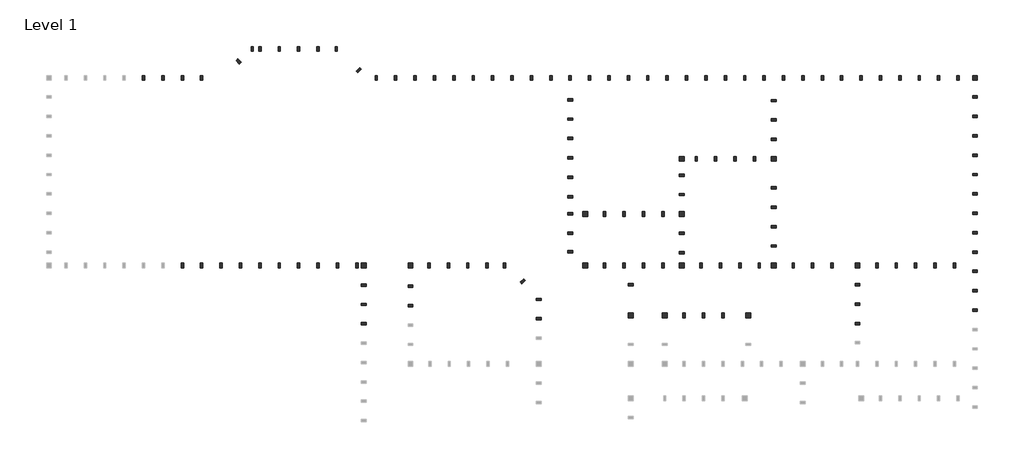
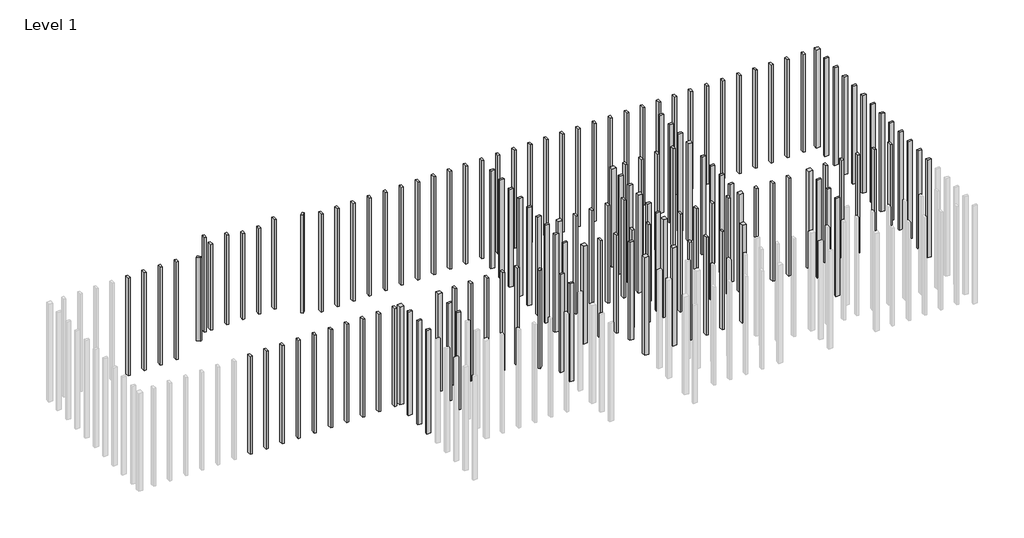
# One storey, part 2 of 2: 143 columns.
"""IFC4 building model written with IfcOpenShell, lengths in millimetres."""

import ifcopenshell
import ifcopenshell.guid

model = None  # the IFC model being written
_history = None  # IfcOwnerHistory: only IFC2X3 demands one
_inside = {}  # id of a spatial element -> (the spatial element, [elements in it])
_under = {}  # id of a project, library or spatial element -> (it, [spatial elements below it])
_declared = {}  # id of a project -> (the project, [libraries it declares])
_typed = {}  # id of a type object -> (the type object, [elements of that type])
_made_of = {}  # id of a material, layer set ... -> (it, [elements and type objects made of it])


def new_model(schema):
    """Start an empty IFC model of exactly this schema.

    Asked for "IFC4X3", IfcOpenShell would pick the latest addendum, in which some entities
    have other attributes; the version numbers below select the first issue.
    IFC2X3 requires an IfcOwnerHistory on every rooted entity: one is made here for all.
    """
    global model, _history
    if schema == "IFC4X3":
        model = ifcopenshell.file(schema_version=(4, 3, 0, 0))
    else:
        model = ifcopenshell.file(schema=schema)
    _inside.clear()
    _under.clear()
    _declared.clear()
    _typed.clear()
    _made_of.clear()
    _history = None
    if model.schema == "IFC2X3":
        org = make("IfcOrganization", Name="unknown")
        user = make(
            "IfcPersonAndOrganization",
            ThePerson=make("IfcPerson", FamilyName="unknown"),
            TheOrganization=org,
        )
        app = make(
            "IfcApplication",
            ApplicationDeveloper=org,
            Version="unknown",
            ApplicationFullName="unknown",
            ApplicationIdentifier="unknown",
        )
        _history = make(
            "IfcOwnerHistory",
            OwningUser=user,
            OwningApplication=app,
            ChangeAction="ADDED",
            CreationDate=0,
        )
    return model


def make(cls, **values):
    """One entity of the class cls with the attributes given. An attribute that is None is left unset."""
    return model.create_entity(
        cls, **{name: value for name, value in values.items() if value is not None}
    )


def rooted(cls, **values):
    """An entity with a GlobalId (a new one), such as an element, a storey or a relation."""
    return make(cls, GlobalId=ifcopenshell.guid.new(), OwnerHistory=_history, **values)


def si_unit(unit_type, name, prefix=None):
    """IfcSIUnit, for example si_unit("LENGTHUNIT", "METRE", prefix="MILLI")."""
    return make("IfcSIUnit", UnitType=unit_type, Prefix=prefix, Name=name)


def assignment(units):
    """IfcUnitAssignment: the units of a project."""
    return None if units is None else make("IfcUnitAssignment", Units=units)


def point(xyz):
    """IfcCartesianPoint."""
    return None if xyz is None else make("IfcCartesianPoint", Coordinates=xyz)


def direction(xyz):
    """IfcDirection."""
    return None if xyz is None else make("IfcDirection", DirectionRatios=xyz)


def frame(location, z_axis=None, x_axis=None):
    """IfcAxis2Placement3D, a coordinate frame: its origin and axes. An axis left out is left unset."""
    return make(
        "IfcAxis2Placement3D",
        Location=point(location),
        Axis=direction(z_axis),
        RefDirection=direction(x_axis),
    )


def origin():
    """The frame at (0, 0, 0) with its axes left unset."""
    return frame((0.0, 0.0, 0.0))


def origin_with_axes():
    """The frame at (0, 0, 0) with the z axis (0, 0, 1) and the x axis (1, 0, 0) written out."""
    return frame((0.0, 0.0, 0.0), z_axis=(0.0, 0.0, 1.0), x_axis=(1.0, 0.0, 0.0))


def place(relative_to, where):
    """IfcLocalPlacement: puts the frame where relative to a parent placement (None: the world)."""
    return make(
        "IfcLocalPlacement", PlacementRelTo=relative_to, RelativePlacement=where
    )


def context(
    kind, dimensions, precision=None, world=None, true_north=None, identifier=None
):
    """IfcGeometricRepresentationContext, for example the 3D "Model" context."""
    return make(
        "IfcGeometricRepresentationContext",
        ContextIdentifier=identifier,
        ContextType=kind,
        CoordinateSpaceDimension=dimensions,
        Precision=precision,
        WorldCoordinateSystem=world,
        TrueNorth=true_north,
    )


def project(units=None, contexts=None):
    """IfcProject with its units and contexts."""
    return rooted(
        "IfcProject",
        Name="project",
        RepresentationContexts=contexts,
        UnitsInContext=assignment(units),
    )


def spatial(cls, under=None, at=None, **own):
    """A site, building, storey or space (cls), placed at a placement, below another one or the project."""
    s = rooted(cls, ObjectPlacement=at, **own)
    if under is not None:
        _under.setdefault(under.id(), (under, []))[1].append(s)
    return s


def polyline(points):
    """IfcPolyline through the points."""
    return make("IfcPolyline", Points=[point(p) for p in points])


def outline(outer, holes=None, kind="AREA"):
    """IfcArbitraryClosedProfileDef: a profile drawn as a closed curve; with holes, ...WithVoids."""
    if holes is None:
        return make("IfcArbitraryClosedProfileDef", ProfileType=kind, OuterCurve=outer)
    return make(
        "IfcArbitraryProfileDefWithVoids",
        ProfileType=kind,
        OuterCurve=outer,
        InnerCurves=holes,
    )


def extrude(swept, where, along, depth):
    """IfcExtrudedAreaSolid: the profile swept, set in the frame where, extruded along a direction by depth."""
    return make(
        "IfcExtrudedAreaSolid",
        SweptArea=swept,
        Position=where,
        ExtrudedDirection=direction(along),
        Depth=depth,
    )


def shape(context_of_items, identifier, shape_type, items):
    """IfcShapeRepresentation: the items that make up one representation, for example the "Body"."""
    return make(
        "IfcShapeRepresentation",
        ContextOfItems=context_of_items,
        RepresentationIdentifier=identifier,
        RepresentationType=shape_type,
        Items=items,
    )


def source(mapping_origin, context_of_items, identifier, shape_type, items):
    """IfcRepresentationMap: a shape defined once, which mapped items show again and again."""
    return make(
        "IfcRepresentationMap",
        MappingOrigin=mapping_origin,
        MappedRepresentation=shape(context_of_items, identifier, shape_type, items),
    )


def transform(
    local_origin,
    x_axis=None,
    y_axis=None,
    z_axis=None,
    scale=None,
    scale2=None,
    scale3=None,
    uniform=True,
):
    """IfcCartesianTransformationOperator3D, or its non-uniform kind. x_axis, y_axis, z_axis: its Axis1, 2, 3."""
    if uniform:
        return make(
            "IfcCartesianTransformationOperator3D",
            Axis1=direction(x_axis),
            Axis2=direction(y_axis),
            LocalOrigin=point(local_origin),
            Scale=scale,
            Axis3=direction(z_axis),
        )
    return make(
        "IfcCartesianTransformationOperator3DnonUniform",
        Axis1=direction(x_axis),
        Axis2=direction(y_axis),
        LocalOrigin=point(local_origin),
        Scale=scale,
        Axis3=direction(z_axis),
        Scale2=scale2,
        Scale3=scale3,
    )


def mapped(mapping_source, mapping_target):
    """IfcMappedItem: shows the shape of a source again, moved by a transform."""
    return make(
        "IfcMappedItem", MappingSource=mapping_source, MappingTarget=mapping_target
    )


def made_of(thing, what):
    """Note that an element or type object is made of a material, layer set ...; save() writes the relation."""
    if what is not None:
        _made_of.setdefault(what.id(), (what, []))[1].append(thing)
    return thing


def element(
    cls,
    number,
    at=None,
    inside=None,
    cuts=None,
    type_object=None,
    material=None,
    context=None,
    identifier="Body",
    shape_type=None,
    held_by="IfcProductDefinitionShape",
    body=None,
    shapes=None,
    **own,
):
    """One element of the class cls, such as IfcWall. Its Tag is "e" and its number.

    at: its placement. inside: the storey or other place that contains it. cuts: it is an
    opening in that element (IfcRelVoidsElement). A single representation is given by context,
    identifier, shape_type and body (its items); several are given by shapes. held_by: the class
    of the entity that holds the representations. save() writes the other relations.
    """
    e = rooted(cls, Tag="e%d" % number, ObjectPlacement=at, **own)
    if body is not None:
        shapes = [shape(context, identifier, shape_type, body)]
    if shapes is not None:
        e.Representation = make(held_by, Representations=shapes)
    if inside is not None:
        _inside.setdefault(inside.id(), (inside, []))[1].append(e)
    if cuts is not None:
        rooted(
            "IfcRelVoidsElement", RelatingBuildingElement=cuts, RelatedOpeningElement=e
        )
    if type_object is not None:
        _typed.setdefault(type_object.id(), (type_object, []))[1].append(e)
    return made_of(e, material)


def aggregate(whole, parts):
    """IfcRelAggregates: a whole, such as a stair, and the parts it consists of."""
    return rooted("IfcRelAggregates", RelatingObject=whole, RelatedObjects=parts)


def save(model, path):
    """Write the relations noted so far, then the file.

    IfcRelAggregates (storeys below a building ...), IfcRelContainedInSpatialStructure (elements
    in a storey), IfcRelDefinesByType, IfcRelAssociatesMaterial and IfcRelDeclares: one each for
    every whole, place, type object, material and project.
    """
    for whole, parts in _under.values():
        aggregate(whole, parts)
    for where, things in _inside.values():
        rooted(
            "IfcRelContainedInSpatialStructure",
            RelatedElements=things,
            RelatingStructure=where,
        )
    for kind, things in _typed.values():
        rooted("IfcRelDefinesByType", RelatedObjects=things, RelatingType=kind)
    for what, things in _made_of.values():
        rooted("IfcRelAssociatesMaterial", RelatedObjects=things, RelatingMaterial=what)
    for by, libraries in _declared.values():
        rooted("IfcRelDeclares", RelatingContext=by, RelatedDefinitions=libraries)
    model.write(path)


def timber_column_65e54e3c(model_context):
    return source(origin(), model_context, "Body", "SweptSolid", [
        extrude(outline(polyline([(25.4, 50.8), (25.4, -50.8), (-25.4, -50.8), (-25.4, 50.8), (25.4, 50.8)])), frame((0.0, 0.0, 50.8), z_axis=(0.0, 0.0, 1.0), x_axis=(1.0, 0.0, 0.0)), (0.0, 0.0, 1.0), 2616.2),
    ])


def timber_column_b7e6a7b9(model_context):
    return source(origin(), model_context, "Body", "SweptSolid", [
        extrude(outline(polyline([(50.8, 50.8), (50.8, -50.8), (-50.8, -50.8), (-50.8, 50.8), (50.8, 50.8)])), frame((0.0, 0.0, 50.8), z_axis=(0.0, 0.0, 1.0), x_axis=(1.0, 0.0, 0.0)), (0.0, 0.0, 1.0), 2616.2),
    ])


def timber_column_c014de30(model_context):
    return source(origin(), model_context, "Body", "SweptSolid", [
        extrude(outline(polyline([(25.4, -50.8), (-25.4, -50.8), (-25.4, 50.8), (25.4, 50.8), (25.4, -50.8)])), frame((0.0, 0.0, 50.8), z_axis=(0.0, 0.0, 1.0), x_axis=(1.0, 0.0, 0.0)), (0.0, 0.0, 1.0), 2616.2),
    ])


def timber_column_7e99ce9a(model_context):
    return source(origin(), model_context, "Body", "SweptSolid", [
        extrude(outline(polyline([(25.4, 50.8), (25.4, -50.8), (-25.4, -50.8), (-25.4, 50.8), (25.4, 50.8)])), origin_with_axes(), (0.0, 0.0, 1.0), 2768.6),
    ])


def timber_column_b6a9144e(model_context):
    return source(origin(), model_context, "Body", "SweptSolid", [
        extrude(outline(polyline([(25.4, 50.8), (25.4, -50.8), (-25.4, -50.8), (-25.4, 50.8), (25.4, 50.8)])), frame((0.0, 0.0, 50.8), z_axis=(0.0, 0.0, 1.0), x_axis=(1.0, 0.0, 0.0)), (0.0, 0.0, 1.0), 2290.1727203),
    ])


model = new_model("IFC4")

# Units and contexts
model_context = context("Model", 3, world=origin())
ifc_project = project(units=[si_unit("LENGTHUNIT", "METRE", prefix="MILLI")], contexts=[model_context])

# Site, building, storey
site = spatial("IfcSite", under=ifc_project)
building = spatial("IfcBuilding", under=site)
storey = spatial("IfcBuildingStorey", under=building, Name="Level 1", Elevation=0.0)

# Columns
placement = place(None, origin())
element("IfcColumn", 1, ObjectType="Timber-Column", at=placement, inside=storey, context=model_context, shape_type="SweptSolid", body=[
    extrude(outline(polyline([(-13305.414829, 5817.3284114), (-13305.414829, 5715.7284114), (-13356.214829, 5715.7284114), (-13356.214829, 5817.3284114), (-13305.414829, 5817.3284114)])), frame((0.0, 0.0, 50.8), z_axis=(0.0, 0.0, 1.0), x_axis=(1.0, 0.0, 0.0)), (0.0, 0.0, 1.0), 2290.1727203),
])
element("IfcColumn", 2, ObjectType="Timber-Column", at=placement, inside=storey, context=model_context, shape_type="SweptSolid", body=[
    extrude(outline(polyline([(-12899.014829, 5817.3284114), (-12899.014829, 5715.7284114), (-12949.814829, 5715.7284114), (-12949.814829, 5817.3284114), (-12899.014829, 5817.3284114)])), frame((0.0, 0.0, 50.8), z_axis=(0.0, 0.0, 1.0), x_axis=(1.0, 0.0, 0.0)), (0.0, 0.0, 1.0), 2391.7727203),
])
element("IfcColumn", 3, ObjectType="Timber-Column", at=placement, inside=storey, context=model_context, shape_type="SweptSolid", body=[
    extrude(outline(polyline([(-13793.9590772, 5557.3841632), (-13722.1170283, 5485.5421142), (-13758.0380528, 5449.6210897), (-13829.8801017, 5521.4631387), (-13793.9590772, 5557.3841632)])), frame((0.0, 0.0, 50.8), z_axis=(0.0, 0.0, 1.0), x_axis=(1.0, 0.0, 0.0)), (0.0, 0.0, 1.0), 2235.2),
])
element("IfcColumn", 4, ObjectType="Timber-Column", at=placement, inside=storey, context=model_context, shape_type="SweptSolid", body=[
    extrude(outline(polyline([(-13464.8030362, 5817.3284114), (-13464.8030362, 5715.7284114), (-13515.6030362, 5715.7284114), (-13515.6030362, 5817.3284114), (-13464.8030362, 5817.3284114)])), frame((0.0, 0.0, 50.8), z_axis=(0.0, 0.0, 1.0), x_axis=(1.0, 0.0, 0.0)), (0.0, 0.0, 1.0), 2528.0077467),
])
element("IfcColumn", 5, ObjectType="Timber-Column", at=placement, inside=storey, context=model_context, shape_type="SweptSolid", body=[
    extrude(outline(polyline([(-11705.214829, 5817.3284114), (-11705.214829, 5715.7284114), (-11756.014829, 5715.7284114), (-11756.014829, 5817.3284114), (-11705.214829, 5817.3284114)])), frame((0.0, 0.0, 50.8), z_axis=(0.0, 0.0, 1.0), x_axis=(1.0, 0.0, 0.0)), (0.0, 0.0, 1.0), 2391.7727203),
])
timber_column_shape = timber_column_65e54e3c(model_context)
element("IfcColumn", 6, ObjectType="Timber-Column", at=placement, inside=storey, context=model_context, shape_type="MappedRepresentation", body=[
    mapped(timber_column_shape, transform((-15769.214829, 5156.9284114, 0.0), x_axis=(1.0, 0.0, 0.0), y_axis=(0.0, 1.0, 0.0), z_axis=(0.0, 0.0, 1.0))),
])
element("IfcColumn", 7, ObjectType="Timber-Column", at=placement, inside=storey, context=model_context, shape_type="MappedRepresentation", body=[
    mapped(timber_column_shape, transform((-15362.814829, 5156.9284114, 0.0), x_axis=(1.0, 0.0, 0.0), y_axis=(0.0, 1.0, 0.0), z_axis=(0.0, 0.0, 1.0))),
])
element("IfcColumn", 8, ObjectType="Timber-Column", at=placement, inside=storey, context=model_context, shape_type="MappedRepresentation", body=[
    mapped(timber_column_shape, transform((-14956.414829, 5156.9284114, 0.0), x_axis=(1.0, 0.0, 0.0), y_axis=(0.0, 1.0, 0.0), z_axis=(0.0, 0.0, 1.0))),
])
element("IfcColumn", 9, ObjectType="Timber-Column", at=placement, inside=storey, context=model_context, shape_type="MappedRepresentation", body=[
    mapped(timber_column_shape, transform((-14550.014829, 5156.9284114, 0.0), x_axis=(1.0, 0.0, 0.0), y_axis=(0.0, 1.0, 0.0), z_axis=(0.0, 0.0, 1.0))),
])
element("IfcColumn", 10, ObjectType="Timber-Column", at=placement, inside=storey, context=model_context, shape_type="MappedRepresentation", body=[
    mapped(timber_column_shape, transform((-10892.414829, 5156.9284114, 0.0), x_axis=(1.0, 0.0, 0.0), y_axis=(0.0, 1.0, 0.0), z_axis=(0.0, 0.0, 1.0))),
])
element("IfcColumn", 11, ObjectType="Timber-Column", at=placement, inside=storey, context=model_context, shape_type="MappedRepresentation", body=[
    mapped(timber_column_shape, transform((-10486.014829, 5156.9284114, 0.0), x_axis=(1.0, 0.0, 0.0), y_axis=(0.0, 1.0, 0.0), z_axis=(0.0, 0.0, 1.0))),
])
element("IfcColumn", 12, ObjectType="Timber-Column", at=placement, inside=storey, context=model_context, shape_type="MappedRepresentation", body=[
    mapped(timber_column_shape, transform((-10079.614829, 5156.9284114, 0.0), x_axis=(1.0, 0.0, 0.0), y_axis=(0.0, 1.0, 0.0), z_axis=(0.0, 0.0, 1.0))),
])
element("IfcColumn", 13, ObjectType="Timber-Column", at=placement, inside=storey, context=model_context, shape_type="MappedRepresentation", body=[
    mapped(timber_column_shape, transform((-9673.214829, 5156.9284114, 0.0), x_axis=(1.0, 0.0, 0.0), y_axis=(0.0, 1.0, 0.0), z_axis=(0.0, 0.0, 1.0))),
])
element("IfcColumn", 14, ObjectType="Timber-Column", at=placement, inside=storey, context=model_context, shape_type="MappedRepresentation", body=[
    mapped(timber_column_shape, transform((-9266.814829, 5156.9284114, 0.0), x_axis=(1.0, 0.0, 0.0), y_axis=(0.0, 1.0, 0.0), z_axis=(0.0, 0.0, 1.0))),
])
element("IfcColumn", 15, ObjectType="Timber-Column", at=placement, inside=storey, context=model_context, shape_type="MappedRepresentation", body=[
    mapped(timber_column_shape, transform((-8860.414829, 5156.9284114, 0.0), x_axis=(1.0, 0.0, 0.0), y_axis=(0.0, 1.0, 0.0), z_axis=(0.0, 0.0, 1.0))),
])
element("IfcColumn", 16, ObjectType="Timber-Column", at=placement, inside=storey, context=model_context, shape_type="MappedRepresentation", body=[
    mapped(timber_column_shape, transform((-8454.014829, 5156.9284114, 0.0), x_axis=(1.0, 0.0, 0.0), y_axis=(0.0, 1.0, 0.0), z_axis=(0.0, 0.0, 1.0))),
])
element("IfcColumn", 17, ObjectType="Timber-Column", at=placement, inside=storey, context=model_context, shape_type="MappedRepresentation", body=[
    mapped(timber_column_shape, transform((-8047.614829, 5156.9284114, 0.0), x_axis=(1.0, 0.0, 0.0), y_axis=(0.0, 1.0, 0.0), z_axis=(0.0, 0.0, 1.0))),
])
element("IfcColumn", 18, ObjectType="Timber-Column", at=placement, inside=storey, context=model_context, shape_type="MappedRepresentation", body=[
    mapped(timber_column_shape, transform((-7641.214829, 5156.9284114, 0.0), x_axis=(1.0, 0.0, 0.0), y_axis=(0.0, 1.0, 0.0), z_axis=(0.0, 0.0, 1.0))),
])
element("IfcColumn", 19, ObjectType="Timber-Column", at=placement, inside=storey, context=model_context, shape_type="MappedRepresentation", body=[
    mapped(timber_column_shape, transform((-7234.814829, 5156.9284114, 0.0), x_axis=(1.0, 0.0, 0.0), y_axis=(0.0, 1.0, 0.0), z_axis=(0.0, 0.0, 1.0))),
])
element("IfcColumn", 20, ObjectType="Timber-Column", at=placement, inside=storey, context=model_context, shape_type="MappedRepresentation", body=[
    mapped(timber_column_shape, transform((-6828.414829, 5156.9284114, 0.0), x_axis=(1.0, 0.0, 0.0), y_axis=(0.0, 1.0, 0.0), z_axis=(0.0, 0.0, 1.0))),
])
element("IfcColumn", 21, ObjectType="Timber-Column", at=placement, inside=storey, context=model_context, shape_type="MappedRepresentation", body=[
    mapped(timber_column_shape, transform((-6422.014829, 5156.9284114, 0.0), x_axis=(1.0, 0.0, 0.0), y_axis=(0.0, 1.0, 0.0), z_axis=(0.0, 0.0, 1.0))),
])
element("IfcColumn", 22, ObjectType="Timber-Column", at=placement, inside=storey, context=model_context, shape_type="MappedRepresentation", body=[
    mapped(timber_column_shape, transform((-6015.614829, 5156.9284114, 0.0), x_axis=(1.0, 0.0, 0.0), y_axis=(0.0, 1.0, 0.0), z_axis=(0.0, 0.0, 1.0))),
])
element("IfcColumn", 23, ObjectType="Timber-Column", at=placement, inside=storey, context=model_context, shape_type="MappedRepresentation", body=[
    mapped(timber_column_shape, transform((-5609.214829, 5156.9284114, 0.0), x_axis=(1.0, 0.0, 0.0), y_axis=(0.0, 1.0, 0.0), z_axis=(0.0, 0.0, 1.0))),
])
element("IfcColumn", 24, ObjectType="Timber-Column", at=placement, inside=storey, context=model_context, shape_type="MappedRepresentation", body=[
    mapped(timber_column_shape, transform((-5202.814829, 5156.9284114, 0.0), x_axis=(1.0, 0.0, 0.0), y_axis=(0.0, 1.0, 0.0), z_axis=(0.0, 0.0, 1.0))),
])
element("IfcColumn", 25, ObjectType="Timber-Column", at=placement, inside=storey, context=model_context, shape_type="MappedRepresentation", body=[
    mapped(timber_column_shape, transform((-4796.414829, 5156.9284114, 0.0), x_axis=(1.0, 0.0, 0.0), y_axis=(0.0, 1.0, 0.0), z_axis=(0.0, 0.0, 1.0))),
])
element("IfcColumn", 26, ObjectType="Timber-Column", at=placement, inside=storey, context=model_context, shape_type="MappedRepresentation", body=[
    mapped(timber_column_shape, transform((-4390.014829, 5156.9284114, 0.0), x_axis=(1.0, 0.0, 0.0), y_axis=(0.0, 1.0, 0.0), z_axis=(0.0, 0.0, 1.0))),
])
element("IfcColumn", 27, ObjectType="Timber-Column", at=placement, inside=storey, context=model_context, shape_type="MappedRepresentation", body=[
    mapped(timber_column_shape, transform((-3983.614829, 5156.9284114, 0.0), x_axis=(1.0, 0.0, 0.0), y_axis=(0.0, 1.0, 0.0), z_axis=(0.0, 0.0, 1.0))),
])
element("IfcColumn", 28, ObjectType="Timber-Column", at=placement, inside=storey, context=model_context, shape_type="MappedRepresentation", body=[
    mapped(timber_column_shape, transform((-3577.214829, 5156.9284114, 0.0), x_axis=(1.0, 0.0, 0.0), y_axis=(0.0, 1.0, 0.0), z_axis=(0.0, 0.0, 1.0))),
])
element("IfcColumn", 29, ObjectType="Timber-Column", at=placement, inside=storey, context=model_context, shape_type="MappedRepresentation", body=[
    mapped(timber_column_shape, transform((-3170.814829, 5156.9284114, 0.0), x_axis=(1.0, 0.0, 0.0), y_axis=(0.0, 1.0, 0.0), z_axis=(0.0, 0.0, 1.0))),
])
element("IfcColumn", 30, ObjectType="Timber-Column", at=placement, inside=storey, context=model_context, shape_type="MappedRepresentation", body=[
    mapped(timber_column_shape, transform((-2764.414829, 5156.9284114, 0.0), x_axis=(1.0, 0.0, 0.0), y_axis=(0.0, 1.0, 0.0), z_axis=(0.0, 0.0, 1.0))),
])
element("IfcColumn", 31, ObjectType="Timber-Column", at=placement, inside=storey, context=model_context, shape_type="MappedRepresentation", body=[
    mapped(timber_column_shape, transform((-2358.014829, 5156.9284114, 0.0), x_axis=(1.0, 0.0, 0.0), y_axis=(0.0, 1.0, 0.0), z_axis=(0.0, 0.0, 1.0))),
])
element("IfcColumn", 32, ObjectType="Timber-Column", at=placement, inside=storey, context=model_context, shape_type="MappedRepresentation", body=[
    mapped(timber_column_shape, transform((-1951.614829, 5156.9284114, 0.0), x_axis=(1.0, 0.0, 0.0), y_axis=(0.0, 1.0, 0.0), z_axis=(0.0, 0.0, 1.0))),
])
element("IfcColumn", 33, ObjectType="Timber-Column", at=placement, inside=storey, context=model_context, shape_type="MappedRepresentation", body=[
    mapped(timber_column_shape, transform((-1545.214829, 5156.9284114, 0.0), x_axis=(1.0, 0.0, 0.0), y_axis=(0.0, 1.0, 0.0), z_axis=(0.0, 0.0, 1.0))),
])
element("IfcColumn", 34, ObjectType="Timber-Column", at=placement, inside=storey, context=model_context, shape_type="MappedRepresentation", body=[
    mapped(timber_column_shape, transform((-1138.814829, 5156.9284114, 0.0), x_axis=(1.0, 0.0, 0.0), y_axis=(0.0, 1.0, 0.0), z_axis=(0.0, 0.0, 1.0))),
])
element("IfcColumn", 35, ObjectType="Timber-Column", at=placement, inside=storey, context=model_context, shape_type="MappedRepresentation", body=[
    mapped(timber_column_shape, transform((-732.414829, 5156.9284114, 0.0), x_axis=(1.0, 0.0, 0.0), y_axis=(0.0, 1.0, 0.0), z_axis=(0.0, 0.0, 1.0))),
])
element("IfcColumn", 36, ObjectType="Timber-Column", at=placement, inside=storey, context=model_context, shape_type="MappedRepresentation", body=[
    mapped(timber_column_shape, transform((-326.014829, 5156.9284114, 0.0), x_axis=(1.0, 0.0, 0.0), y_axis=(0.0, 1.0, 0.0), z_axis=(0.0, 0.0, 1.0))),
])
element("IfcColumn", 37, ObjectType="Timber-Column", at=placement, inside=storey, context=model_context, shape_type="MappedRepresentation", body=[
    mapped(timber_column_shape, transform((80.385171, 5156.9284114, 0.0), x_axis=(1.0, 0.0, 0.0), y_axis=(0.0, 1.0, 0.0), z_axis=(0.0, 0.0, 1.0))),
])
element("IfcColumn", 38, ObjectType="Timber-Column", at=placement, inside=storey, context=model_context, shape_type="MappedRepresentation", body=[
    mapped(timber_column_shape, transform((486.785171, 5156.9284114, 0.0), x_axis=(1.0, 0.0, 0.0), y_axis=(0.0, 1.0, 0.0), z_axis=(0.0, 0.0, 1.0))),
])
element("IfcColumn", 39, ObjectType="Timber-Column", at=placement, inside=storey, context=model_context, shape_type="MappedRepresentation", body=[
    mapped(timber_column_shape, transform((893.185171, 5156.9284114, 0.0), x_axis=(1.0, 0.0, 0.0), y_axis=(0.0, 1.0, 0.0), z_axis=(0.0, 0.0, 1.0))),
])
element("IfcColumn", 40, ObjectType="Timber-Column", at=placement, inside=storey, context=model_context, shape_type="MappedRepresentation", body=[
    mapped(timber_column_shape, transform((1299.585171, 5156.9284114, 0.0), x_axis=(1.0, 0.0, 0.0), y_axis=(0.0, 1.0, 0.0), z_axis=(0.0, 0.0, 1.0))),
])
element("IfcColumn", 41, ObjectType="Timber-Column", at=placement, inside=storey, context=model_context, shape_type="MappedRepresentation", body=[
    mapped(timber_column_shape, transform((-11298.814829, 1226.2784114, 0.0), x_axis=(1.0, 0.0, 0.0), y_axis=(0.0, 1.0, 0.0), z_axis=(0.0, 0.0, 1.0))),
])
element("IfcColumn", 42, ObjectType="Timber-Column", at=placement, inside=storey, context=model_context, shape_type="MappedRepresentation", body=[
    mapped(timber_column_shape, transform((-11705.214829, 1226.2784114, 0.0), x_axis=(1.0, 0.0, 0.0), y_axis=(0.0, 1.0, 0.0), z_axis=(0.0, 0.0, 1.0))),
])
element("IfcColumn", 43, ObjectType="Timber-Column", at=placement, inside=storey, context=model_context, shape_type="MappedRepresentation", body=[
    mapped(timber_column_shape, transform((-12111.614829, 1226.2784114, 0.0), x_axis=(1.0, 0.0, 0.0), y_axis=(0.0, 1.0, 0.0), z_axis=(0.0, 0.0, 1.0))),
])
element("IfcColumn", 44, ObjectType="Timber-Column", at=placement, inside=storey, context=model_context, shape_type="MappedRepresentation", body=[
    mapped(timber_column_shape, transform((-12518.014829, 1226.2784114, 0.0), x_axis=(1.0, 0.0, 0.0), y_axis=(0.0, 1.0, 0.0), z_axis=(0.0, 0.0, 1.0))),
])
element("IfcColumn", 45, ObjectType="Timber-Column", at=placement, inside=storey, context=model_context, shape_type="MappedRepresentation", body=[
    mapped(timber_column_shape, transform((-12924.414829, 1226.2784114, 0.0), x_axis=(1.0, 0.0, 0.0), y_axis=(0.0, 1.0, 0.0), z_axis=(0.0, 0.0, 1.0))),
])
element("IfcColumn", 46, ObjectType="Timber-Column", at=placement, inside=storey, context=model_context, shape_type="MappedRepresentation", body=[
    mapped(timber_column_shape, transform((-13330.814829, 1226.2784114, 0.0), x_axis=(1.0, 0.0, 0.0), y_axis=(0.0, 1.0, 0.0), z_axis=(0.0, 0.0, 1.0))),
])
element("IfcColumn", 47, ObjectType="Timber-Column", at=placement, inside=storey, context=model_context, shape_type="MappedRepresentation", body=[
    mapped(timber_column_shape, transform((-13737.214829, 1226.2784114, 0.0), x_axis=(1.0, 0.0, 0.0), y_axis=(0.0, 1.0, 0.0), z_axis=(0.0, 0.0, 1.0))),
])
element("IfcColumn", 48, ObjectType="Timber-Column", at=placement, inside=storey, context=model_context, shape_type="MappedRepresentation", body=[
    mapped(timber_column_shape, transform((-14143.614829, 1226.2784114, 0.0), x_axis=(1.0, 0.0, 0.0), y_axis=(0.0, 1.0, 0.0), z_axis=(0.0, 0.0, 1.0))),
])
element("IfcColumn", 49, ObjectType="Timber-Column", at=placement, inside=storey, context=model_context, shape_type="MappedRepresentation", body=[
    mapped(timber_column_shape, transform((-14550.014829, 1226.2784114, 0.0), x_axis=(1.0, 0.0, 0.0), y_axis=(0.0, 1.0, 0.0), z_axis=(0.0, 0.0, 1.0))),
])
element("IfcColumn", 50, ObjectType="Timber-Column", at=placement, inside=storey, context=model_context, shape_type="MappedRepresentation", body=[
    mapped(timber_column_shape, transform((-14956.414829, 1226.2784114, 0.0), x_axis=(1.0, 0.0, 0.0), y_axis=(0.0, 1.0, 0.0), z_axis=(0.0, 0.0, 1.0))),
])
element("IfcColumn", 51, ObjectType="Timber-Column", at=placement, inside=storey, context=model_context, shape_type="MappedRepresentation", body=[
    mapped(timber_column_shape, transform((-11259.6474151, 5320.9609974, 0.0), x_axis=(0.7071067811865546, -0.7071067811865406, 0.0), y_axis=(0.7071067811865406, 0.7071067811865546, 0.0), z_axis=(0.0, 0.0, 1.0))),
])
element("IfcColumn", 52, ObjectType="Timber-Column", at=placement, inside=storey, context=model_context, shape_type="MappedRepresentation", body=[
    mapped(timber_column_shape, transform((-6828.414829, 4699.7284114, 0.0), x_axis=(0.0, 1.0, 0.0), y_axis=(-1.0, 0.0, 0.0), z_axis=(0.0, 0.0, 1.0))),
])
element("IfcColumn", 53, ObjectType="Timber-Column", at=placement, inside=storey, context=model_context, shape_type="MappedRepresentation", body=[
    mapped(timber_column_shape, transform((-6828.414829, 4293.3284114, 0.0), x_axis=(0.0, 1.0, 0.0), y_axis=(-1.0, 0.0, 0.0), z_axis=(0.0, 0.0, 1.0))),
])
element("IfcColumn", 54, ObjectType="Timber-Column", at=placement, inside=storey, context=model_context, shape_type="MappedRepresentation", body=[
    mapped(timber_column_shape, transform((-6828.414829, 3886.9284114, 0.0), x_axis=(0.0, 1.0, 0.0), y_axis=(-1.0, 0.0, 0.0), z_axis=(0.0, 0.0, 1.0))),
])
element("IfcColumn", 55, ObjectType="Timber-Column", at=placement, inside=storey, context=model_context, shape_type="MappedRepresentation", body=[
    mapped(timber_column_shape, transform((-6828.414829, 3480.5284114, 0.0), x_axis=(0.0, 1.0, 0.0), y_axis=(-1.0, 0.0, 0.0), z_axis=(0.0, 0.0, 1.0))),
])
element("IfcColumn", 56, ObjectType="Timber-Column", at=placement, inside=storey, context=model_context, shape_type="MappedRepresentation", body=[
    mapped(timber_column_shape, transform((-6828.414829, 3074.1284114, 0.0), x_axis=(0.0, 1.0, 0.0), y_axis=(-1.0, 0.0, 0.0), z_axis=(0.0, 0.0, 1.0))),
])
element("IfcColumn", 57, ObjectType="Timber-Column", at=placement, inside=storey, context=model_context, shape_type="MappedRepresentation", body=[
    mapped(timber_column_shape, transform((-6828.414829, 2667.7284114, 0.0), x_axis=(0.0, 1.0, 0.0), y_axis=(-1.0, 0.0, 0.0), z_axis=(0.0, 0.0, 1.0))),
])
element("IfcColumn", 58, ObjectType="Timber-Column", at=placement, inside=storey, context=model_context, shape_type="MappedRepresentation", body=[
    mapped(timber_column_shape, transform((-6828.414829, 2305.7784114, 0.0), x_axis=(0.0, 1.0, 0.0), y_axis=(-1.0, 0.0, 0.0), z_axis=(0.0, 0.0, 1.0))),
])
element("IfcColumn", 59, ObjectType="Timber-Column", at=placement, inside=storey, context=model_context, shape_type="MappedRepresentation", body=[
    mapped(timber_column_shape, transform((-6828.414829, 1899.3784114, 0.0), x_axis=(0.0, 1.0, 0.0), y_axis=(-1.0, 0.0, 0.0), z_axis=(0.0, 0.0, 1.0))),
])
element("IfcColumn", 60, ObjectType="Timber-Column", at=placement, inside=storey, context=model_context, shape_type="MappedRepresentation", body=[
    mapped(timber_column_shape, transform((-6828.414829, 1516.0125093, 0.0), x_axis=(0.0, 1.0, 0.0), y_axis=(-1.0, 0.0, 0.0), z_axis=(0.0, 0.0, 1.0))),
])
element("IfcColumn", 61, ObjectType="Timber-Column", at=placement, inside=storey, context=model_context, shape_type="MappedRepresentation", body=[
    mapped(timber_column_shape, transform((-6106.8807311, 1226.2784114, 0.0), x_axis=(-1.0, 0.0, 0.0), y_axis=(0.0, -1.0, 0.0), z_axis=(0.0, 0.0, 1.0))),
])
element("IfcColumn", 62, ObjectType="Timber-Column", at=placement, inside=storey, context=model_context, shape_type="MappedRepresentation", body=[
    mapped(timber_column_shape, transform((-5700.4807311, 1226.2784114, 0.0), x_axis=(-1.0, 0.0, 0.0), y_axis=(0.0, -1.0, 0.0), z_axis=(0.0, 0.0, 1.0))),
])
element("IfcColumn", 63, ObjectType="Timber-Column", at=placement, inside=storey, context=model_context, shape_type="MappedRepresentation", body=[
    mapped(timber_column_shape, transform((-5294.0807311, 1226.2784114, 0.0), x_axis=(-1.0, 0.0, 0.0), y_axis=(0.0, -1.0, 0.0), z_axis=(0.0, 0.0, 1.0))),
])
element("IfcColumn", 64, ObjectType="Timber-Column", at=placement, inside=storey, context=model_context, shape_type="MappedRepresentation", body=[
    mapped(timber_column_shape, transform((-4887.6807311, 1226.2784114, 0.0), x_axis=(-1.0, 0.0, 0.0), y_axis=(0.0, -1.0, 0.0), z_axis=(0.0, 0.0, 1.0))),
])
element("IfcColumn", 65, ObjectType="Timber-Column", at=placement, inside=storey, context=model_context, shape_type="MappedRepresentation", body=[
    mapped(timber_column_shape, transform((-4085.214829, 1226.2784114, 0.0), x_axis=(-1.0, 0.0, 0.0), y_axis=(0.0, -1.0, 0.0), z_axis=(0.0, 0.0, 1.0))),
])
element("IfcColumn", 66, ObjectType="Timber-Column", at=placement, inside=storey, context=model_context, shape_type="MappedRepresentation", body=[
    mapped(timber_column_shape, transform((-3678.814829, 1226.2784114, 0.0), x_axis=(-1.0, 0.0, 0.0), y_axis=(0.0, -1.0, 0.0), z_axis=(0.0, 0.0, 1.0))),
])
element("IfcColumn", 67, ObjectType="Timber-Column", at=placement, inside=storey, context=model_context, shape_type="MappedRepresentation", body=[
    mapped(timber_column_shape, transform((-3272.414829, 1226.2784114, 0.0), x_axis=(-1.0, 0.0, 0.0), y_axis=(0.0, -1.0, 0.0), z_axis=(0.0, 0.0, 1.0))),
])
element("IfcColumn", 68, ObjectType="Timber-Column", at=placement, inside=storey, context=model_context, shape_type="MappedRepresentation", body=[
    mapped(timber_column_shape, transform((-2866.014829, 1226.2784114, 0.0), x_axis=(-1.0, 0.0, 0.0), y_axis=(0.0, -1.0, 0.0), z_axis=(0.0, 0.0, 1.0))),
])
element("IfcColumn", 69, ObjectType="Timber-Column", at=placement, inside=storey, context=model_context, shape_type="MappedRepresentation", body=[
    mapped(timber_column_shape, transform((-2154.814829, 1226.2784114, 0.0), x_axis=(-1.0, 0.0, 0.0), y_axis=(0.0, -1.0, 0.0), z_axis=(0.0, 0.0, 1.0))),
])
element("IfcColumn", 70, ObjectType="Timber-Column", at=placement, inside=storey, context=model_context, shape_type="MappedRepresentation", body=[
    mapped(timber_column_shape, transform((-1748.414829, 1226.2784114, 0.0), x_axis=(-1.0, 0.0, 0.0), y_axis=(0.0, -1.0, 0.0), z_axis=(0.0, 0.0, 1.0))),
])
element("IfcColumn", 71, ObjectType="Timber-Column", at=placement, inside=storey, context=model_context, shape_type="MappedRepresentation", body=[
    mapped(timber_column_shape, transform((-1342.014829, 1226.2784114, 0.0), x_axis=(-1.0, 0.0, 0.0), y_axis=(0.0, -1.0, 0.0), z_axis=(0.0, 0.0, 1.0))),
])
element("IfcColumn", 72, ObjectType="Timber-Column", at=placement, inside=storey, context=model_context, shape_type="MappedRepresentation", body=[
    mapped(timber_column_shape, transform((-402.214829, 1226.2784114, 0.0), x_axis=(-1.0, 0.0, 0.0), y_axis=(0.0, -1.0, 0.0), z_axis=(0.0, 0.0, 1.0))),
])
element("IfcColumn", 73, ObjectType="Timber-Column", at=placement, inside=storey, context=model_context, shape_type="MappedRepresentation", body=[
    mapped(timber_column_shape, transform((4.185171, 1226.2784114, 0.0), x_axis=(-1.0, 0.0, 0.0), y_axis=(0.0, -1.0, 0.0), z_axis=(0.0, 0.0, 1.0))),
])
element("IfcColumn", 74, ObjectType="Timber-Column", at=placement, inside=storey, context=model_context, shape_type="MappedRepresentation", body=[
    mapped(timber_column_shape, transform((410.585171, 1226.2784114, 0.0), x_axis=(-1.0, 0.0, 0.0), y_axis=(0.0, -1.0, 0.0), z_axis=(0.0, 0.0, 1.0))),
])
element("IfcColumn", 75, ObjectType="Timber-Column", at=placement, inside=storey, context=model_context, shape_type="MappedRepresentation", body=[
    mapped(timber_column_shape, transform((816.985171, 1226.2784114, 0.0), x_axis=(-1.0, 0.0, 0.0), y_axis=(0.0, -1.0, 0.0), z_axis=(0.0, 0.0, 1.0))),
])
element("IfcColumn", 76, ObjectType="Timber-Column", at=placement, inside=storey, context=model_context, shape_type="MappedRepresentation", body=[
    mapped(timber_column_shape, transform((1223.385171, 1226.2784114, 0.0), x_axis=(-1.0, 0.0, 0.0), y_axis=(0.0, -1.0, 0.0), z_axis=(0.0, 0.0, 1.0))),
])
element("IfcColumn", 77, ObjectType="Timber-Column", at=placement, inside=storey, context=model_context, shape_type="MappedRepresentation", body=[
    mapped(timber_column_shape, transform((-6106.8807311, 2305.7784114, 0.0), x_axis=(-1.0, 0.0, 0.0), y_axis=(0.0, -1.0, 0.0), z_axis=(0.0, 0.0, 1.0))),
])
element("IfcColumn", 78, ObjectType="Timber-Column", at=placement, inside=storey, context=model_context, shape_type="MappedRepresentation", body=[
    mapped(timber_column_shape, transform((-5700.4807311, 2305.7784114, 0.0), x_axis=(-1.0, 0.0, 0.0), y_axis=(0.0, -1.0, 0.0), z_axis=(0.0, 0.0, 1.0))),
])
element("IfcColumn", 79, ObjectType="Timber-Column", at=placement, inside=storey, context=model_context, shape_type="MappedRepresentation", body=[
    mapped(timber_column_shape, transform((-5294.0807311, 2305.7784114, 0.0), x_axis=(-1.0, 0.0, 0.0), y_axis=(0.0, -1.0, 0.0), z_axis=(0.0, 0.0, 1.0))),
])
element("IfcColumn", 80, ObjectType="Timber-Column", at=placement, inside=storey, context=model_context, shape_type="MappedRepresentation", body=[
    mapped(timber_column_shape, transform((-4887.6807311, 2305.7784114, 0.0), x_axis=(-1.0, 0.0, 0.0), y_axis=(0.0, -1.0, 0.0), z_axis=(0.0, 0.0, 1.0))),
])
element("IfcColumn", 81, ObjectType="Timber-Column", at=placement, inside=storey, context=model_context, shape_type="MappedRepresentation", body=[
    mapped(timber_column_shape, transform((-4491.614829, 1899.3784114, 0.0), x_axis=(0.0, 1.0, 0.0), y_axis=(-1.0, 0.0, 0.0), z_axis=(0.0, 0.0, 1.0))),
])
element("IfcColumn", 82, ObjectType="Timber-Column", at=placement, inside=storey, context=model_context, shape_type="MappedRepresentation", body=[
    mapped(timber_column_shape, transform((-4491.614829, 1492.9784114, 0.0), x_axis=(0.0, 1.0, 0.0), y_axis=(-1.0, 0.0, 0.0), z_axis=(0.0, 0.0, 1.0))),
])
element("IfcColumn", 83, ObjectType="Timber-Column", at=placement, inside=storey, context=model_context, shape_type="MappedRepresentation", body=[
    mapped(timber_column_shape, transform((-4491.614829, 2712.1784114, 0.0), x_axis=(0.0, 1.0, 0.0), y_axis=(-1.0, 0.0, 0.0), z_axis=(0.0, 0.0, 1.0))),
])
element("IfcColumn", 84, ObjectType="Timber-Column", at=placement, inside=storey, context=model_context, shape_type="MappedRepresentation", body=[
    mapped(timber_column_shape, transform((-4491.614829, 3118.5784114, 0.0), x_axis=(0.0, 1.0, 0.0), y_axis=(-1.0, 0.0, 0.0), z_axis=(0.0, 0.0, 1.0))),
])
element("IfcColumn", 85, ObjectType="Timber-Column", at=placement, inside=storey, context=model_context, shape_type="MappedRepresentation", body=[
    mapped(timber_column_shape, transform((-2967.614829, 3461.4784114, 0.0), x_axis=(1.0, 0.0, 0.0), y_axis=(0.0, 1.0, 0.0), z_axis=(0.0, 0.0, 1.0))),
])
element("IfcColumn", 86, ObjectType="Timber-Column", at=placement, inside=storey, context=model_context, shape_type="MappedRepresentation", body=[
    mapped(timber_column_shape, transform((-3374.014829, 3461.4784114, 0.0), x_axis=(1.0, 0.0, 0.0), y_axis=(0.0, 1.0, 0.0), z_axis=(0.0, 0.0, 1.0))),
])
element("IfcColumn", 87, ObjectType="Timber-Column", at=placement, inside=storey, context=model_context, shape_type="MappedRepresentation", body=[
    mapped(timber_column_shape, transform((-3780.414829, 3461.4784114, 0.0), x_axis=(1.0, 0.0, 0.0), y_axis=(0.0, 1.0, 0.0), z_axis=(0.0, 0.0, 1.0))),
])
element("IfcColumn", 88, ObjectType="Timber-Column", at=placement, inside=storey, context=model_context, shape_type="MappedRepresentation", body=[
    mapped(timber_column_shape, transform((-4186.814829, 3461.4784114, 0.0), x_axis=(1.0, 0.0, 0.0), y_axis=(0.0, 1.0, 0.0), z_axis=(0.0, 0.0, 1.0))),
])
element("IfcColumn", 89, ObjectType="Timber-Column", at=placement, inside=storey, context=model_context, shape_type="MappedRepresentation", body=[
    mapped(timber_column_shape, transform((-2561.214829, 1632.6784114, 0.0), x_axis=(0.0, 1.0, 0.0), y_axis=(-1.0, 0.0, 0.0), z_axis=(0.0, 0.0, 1.0))),
])
element("IfcColumn", 90, ObjectType="Timber-Column", at=placement, inside=storey, context=model_context, shape_type="MappedRepresentation", body=[
    mapped(timber_column_shape, transform((-2561.214829, 2039.0784114, 0.0), x_axis=(0.0, 1.0, 0.0), y_axis=(-1.0, 0.0, 0.0), z_axis=(0.0, 0.0, 1.0))),
])
element("IfcColumn", 91, ObjectType="Timber-Column", at=placement, inside=storey, context=model_context, shape_type="MappedRepresentation", body=[
    mapped(timber_column_shape, transform((-2561.214829, 2445.4784114, 0.0), x_axis=(0.0, 1.0, 0.0), y_axis=(-1.0, 0.0, 0.0), z_axis=(0.0, 0.0, 1.0))),
])
element("IfcColumn", 92, ObjectType="Timber-Column", at=placement, inside=storey, context=model_context, shape_type="MappedRepresentation", body=[
    mapped(timber_column_shape, transform((-2561.214829, 2851.8784114, 0.0), x_axis=(0.0, 1.0, 0.0), y_axis=(-1.0, 0.0, 0.0), z_axis=(0.0, 0.0, 1.0))),
])
element("IfcColumn", 93, ObjectType="Timber-Column", at=placement, inside=storey, context=model_context, shape_type="MappedRepresentation", body=[
    mapped(timber_column_shape, transform((-8203.998927, 1226.2784114, 0.0), x_axis=(1.0, 0.0, 0.0), y_axis=(0.0, 1.0, 0.0), z_axis=(0.0, 0.0, 1.0))),
])
element("IfcColumn", 94, ObjectType="Timber-Column", at=placement, inside=storey, context=model_context, shape_type="MappedRepresentation", body=[
    mapped(timber_column_shape, transform((-8568.7720585, 1226.2784114, 0.0), x_axis=(1.0, 0.0, 0.0), y_axis=(0.0, 1.0, 0.0), z_axis=(0.0, 0.0, 1.0))),
])
element("IfcColumn", 95, ObjectType="Timber-Column", at=placement, inside=storey, context=model_context, shape_type="MappedRepresentation", body=[
    mapped(timber_column_shape, transform((-8975.1720585, 1226.2784114, 0.0), x_axis=(1.0, 0.0, 0.0), y_axis=(0.0, 1.0, 0.0), z_axis=(0.0, 0.0, 1.0))),
])
element("IfcColumn", 96, ObjectType="Timber-Column", at=placement, inside=storey, context=model_context, shape_type="MappedRepresentation", body=[
    mapped(timber_column_shape, transform((-9381.5720585, 1226.2784114, 0.0), x_axis=(1.0, 0.0, 0.0), y_axis=(0.0, 1.0, 0.0), z_axis=(0.0, 0.0, 1.0))),
])
element("IfcColumn", 97, ObjectType="Timber-Column", at=placement, inside=storey, context=model_context, shape_type="MappedRepresentation", body=[
    mapped(timber_column_shape, transform((-9787.9720585, 1226.2784114, 0.0), x_axis=(1.0, 0.0, 0.0), y_axis=(0.0, 1.0, 0.0), z_axis=(0.0, 0.0, 1.0))),
])
element("IfcColumn", 98, ObjectType="Timber-Column", at=placement, inside=storey, context=model_context, shape_type="MappedRepresentation", body=[
    mapped(timber_column_shape, transform((-7488.814829, 511.0943134, 0.0), x_axis=(0.0, 1.0, 0.0), y_axis=(-1.0, 0.0, 0.0), z_axis=(0.0, 0.0, 1.0))),
])
element("IfcColumn", 99, ObjectType="Timber-Column", at=placement, inside=storey, context=model_context, shape_type="MappedRepresentation", body=[
    mapped(timber_column_shape, transform((-7488.814829, 104.6943134, 0.0), x_axis=(0.0, 1.0, 0.0), y_axis=(-1.0, 0.0, 0.0), z_axis=(0.0, 0.0, 1.0))),
])
element("IfcColumn", 100, ObjectType="Timber-Column", at=placement, inside=storey, context=model_context, shape_type="MappedRepresentation", body=[
    mapped(timber_column_shape, transform((-7822.589312, 891.3108454, 0.0), x_axis=(0.7071067811865449, -0.70710678118655, 0.0), y_axis=(0.70710678118655, 0.7071067811865449, 0.0), z_axis=(0.0, 0.0, 1.0))),
])
element("IfcColumn", 101, ObjectType="Timber-Column", at=placement, inside=storey, context=model_context, shape_type="MappedRepresentation", body=[
    mapped(timber_column_shape, transform((-2561.214829, 3867.8784114, 0.0), x_axis=(0.0, 1.0, 0.0), y_axis=(-1.0, 0.0, 0.0), z_axis=(0.0, 0.0, 1.0))),
])
element("IfcColumn", 102, ObjectType="Timber-Column", at=placement, inside=storey, context=model_context, shape_type="MappedRepresentation", body=[
    mapped(timber_column_shape, transform((-2561.214829, 4274.2784114, 0.0), x_axis=(0.0, 1.0, 0.0), y_axis=(-1.0, 0.0, 0.0), z_axis=(0.0, 0.0, 1.0))),
])
element("IfcColumn", 103, ObjectType="Timber-Column", at=placement, inside=storey, context=model_context, shape_type="MappedRepresentation", body=[
    mapped(timber_column_shape, transform((-2561.214829, 4680.6784114, 0.0), x_axis=(0.0, 1.0, 0.0), y_axis=(-1.0, 0.0, 0.0), z_axis=(0.0, 0.0, 1.0))),
])
element("IfcColumn", 104, ObjectType="Timber-Column", at=placement, inside=storey, context=model_context, shape_type="MappedRepresentation", body=[
    mapped(timber_column_shape, transform((-10175.1225949, 381.7284114, 0.0), x_axis=(0.0, 1.0, 0.0), y_axis=(-1.0, 0.0, 0.0), z_axis=(0.0, 0.0, 1.0))),
])
element("IfcColumn", 105, ObjectType="Timber-Column", at=placement, inside=storey, context=model_context, shape_type="MappedRepresentation", body=[
    mapped(timber_column_shape, transform((-10175.1225949, 788.1284114, 0.0), x_axis=(0.0, 1.0, 0.0), y_axis=(-1.0, 0.0, 0.0), z_axis=(0.0, 0.0, 1.0))),
])
element("IfcColumn", 106, ObjectType="Timber-Column", at=placement, inside=storey, context=model_context, shape_type="MappedRepresentation", body=[
    mapped(timber_column_shape, transform((-5558.414829, 819.8784114, 0.0), x_axis=(0.0, 1.0, 0.0), y_axis=(-1.0, 0.0, 0.0), z_axis=(0.0, 0.0, 1.0))),
])
element("IfcColumn", 107, ObjectType="Timber-Column", at=placement, inside=storey, context=model_context, shape_type="MappedRepresentation", body=[
    mapped(timber_column_shape, transform((-4440.814829, 178.5284114, 0.0), x_axis=(-1.0, 0.0, 0.0), y_axis=(0.0, -1.0, 0.0), z_axis=(0.0, 0.0, 1.0))),
])
element("IfcColumn", 108, ObjectType="Timber-Column", at=placement, inside=storey, context=model_context, shape_type="MappedRepresentation", body=[
    mapped(timber_column_shape, transform((-4034.414829, 178.5284114, 0.0), x_axis=(-1.0, 0.0, 0.0), y_axis=(0.0, -1.0, 0.0), z_axis=(0.0, 0.0, 1.0))),
])
element("IfcColumn", 109, ObjectType="Timber-Column", at=placement, inside=storey, context=model_context, shape_type="MappedRepresentation", body=[
    mapped(timber_column_shape, transform((-3628.014829, 178.5284114, 0.0), x_axis=(-1.0, 0.0, 0.0), y_axis=(0.0, -1.0, 0.0), z_axis=(0.0, 0.0, 1.0))),
])
element("IfcColumn", 110, ObjectType="Timber-Column", at=placement, inside=storey, context=model_context, shape_type="MappedRepresentation", body=[
    mapped(timber_column_shape, transform((-808.614829, 819.8784114, 0.0), x_axis=(0.0, 1.0, 0.0), y_axis=(-1.0, 0.0, 0.0), z_axis=(0.0, 0.0, 1.0))),
])
element("IfcColumn", 111, ObjectType="Timber-Column", at=placement, inside=storey, context=model_context, shape_type="MappedRepresentation", body=[
    mapped(timber_column_shape, transform((-808.614829, 413.4784114, 0.0), x_axis=(0.0, 1.0, 0.0), y_axis=(-1.0, 0.0, 0.0), z_axis=(0.0, 0.0, 1.0))),
])
element("IfcColumn", 112, ObjectType="Timber-Column", at=placement, inside=storey, context=model_context, shape_type="MappedRepresentation", body=[
    mapped(timber_column_shape, transform((-808.614829, 7.0784114, 0.0), x_axis=(0.0, 1.0, 0.0), y_axis=(-1.0, 0.0, 0.0), z_axis=(0.0, 0.0, 1.0))),
])
timber_column_2_shape = timber_column_b7e6a7b9(model_context)
element("IfcColumn", 113, ObjectType="Timber-Column", at=placement, inside=storey, context=model_context, shape_type="MappedRepresentation", body=[
    mapped(timber_column_2_shape, transform((-11152.764829, 1226.2784114, 0.0), x_axis=(1.0, 0.0, 0.0), y_axis=(0.0, 1.0, 0.0), z_axis=(0.0, 0.0, 1.0))),
])
element("IfcColumn", 114, ObjectType="Timber-Column", at=placement, inside=storey, context=model_context, shape_type="MappedRepresentation", body=[
    mapped(timber_column_2_shape, transform((1655.185171, 5156.9284114, 0.0), x_axis=(1.0, 0.0, 0.0), y_axis=(0.0, 1.0, 0.0), z_axis=(0.0, 0.0, 1.0))),
])
element("IfcColumn", 115, ObjectType="Timber-Column", at=placement, inside=storey, context=model_context, shape_type="MappedRepresentation", body=[
    mapped(timber_column_2_shape, transform((-4491.614829, 3461.4784114, 0.0), x_axis=(1.0, 0.0, 0.0), y_axis=(0.0, 1.0, 0.0), z_axis=(0.0, 0.0, 1.0))),
])
element("IfcColumn", 116, ObjectType="Timber-Column", at=placement, inside=storey, context=model_context, shape_type="MappedRepresentation", body=[
    mapped(timber_column_2_shape, transform((-4491.614829, 2305.7784114, 0.0), x_axis=(1.0, 0.0, 0.0), y_axis=(0.0, 1.0, 0.0), z_axis=(0.0, 0.0, 1.0))),
])
element("IfcColumn", 117, ObjectType="Timber-Column", at=placement, inside=storey, context=model_context, shape_type="MappedRepresentation", body=[
    mapped(timber_column_2_shape, transform((-4491.614829, 1226.2784114, 0.0), x_axis=(1.0, 0.0, 0.0), y_axis=(0.0, 1.0, 0.0), z_axis=(0.0, 0.0, 1.0))),
])
element("IfcColumn", 118, ObjectType="Timber-Column", at=placement, inside=storey, context=model_context, shape_type="MappedRepresentation", body=[
    mapped(timber_column_2_shape, transform((-2561.214829, 1226.2784114, 0.0), x_axis=(1.0, 0.0, 0.0), y_axis=(0.0, 1.0, 0.0), z_axis=(0.0, 0.0, 1.0))),
])
element("IfcColumn", 119, ObjectType="Timber-Column", at=placement, inside=storey, context=model_context, shape_type="MappedRepresentation", body=[
    mapped(timber_column_2_shape, transform((-2561.214829, 3461.4784114, 0.0), x_axis=(1.0, 0.0, 0.0), y_axis=(0.0, 1.0, 0.0), z_axis=(0.0, 0.0, 1.0))),
])
element("IfcColumn", 120, ObjectType="Timber-Column", at=placement, inside=storey, context=model_context, shape_type="MappedRepresentation", body=[
    mapped(timber_column_2_shape, transform((-6513.2807311, 1226.2784114, 0.0), x_axis=(1.0, 0.0, 0.0), y_axis=(0.0, 1.0, 0.0), z_axis=(0.0, 0.0, 1.0))),
])
element("IfcColumn", 121, ObjectType="Timber-Column", at=placement, inside=storey, context=model_context, shape_type="MappedRepresentation", body=[
    mapped(timber_column_2_shape, transform((-6513.2807311, 2305.7784114, 0.0), x_axis=(1.0, 0.0, 0.0), y_axis=(0.0, 1.0, 0.0), z_axis=(0.0, 0.0, 1.0))),
])
element("IfcColumn", 122, ObjectType="Timber-Column", at=placement, inside=storey, context=model_context, shape_type="MappedRepresentation", body=[
    mapped(timber_column_2_shape, transform((-808.614829, 1226.2784114, 0.0), x_axis=(1.0, 0.0, 0.0), y_axis=(0.0, 1.0, 0.0), z_axis=(0.0, 0.0, 1.0))),
])
element("IfcColumn", 123, ObjectType="Timber-Column", at=placement, inside=storey, context=model_context, shape_type="MappedRepresentation", body=[
    mapped(timber_column_2_shape, transform((-5558.414829, 178.5284114, 0.0), x_axis=(1.0, 0.0, 0.0), y_axis=(0.0, 1.0, 0.0), z_axis=(0.0, 0.0, 1.0))),
])
element("IfcColumn", 124, ObjectType="Timber-Column", at=placement, inside=storey, context=model_context, shape_type="MappedRepresentation", body=[
    mapped(timber_column_2_shape, transform((-10174.864829, 1226.2784114, 0.0), x_axis=(1.0, 0.0, 0.0), y_axis=(0.0, 1.0, 0.0), z_axis=(0.0, 0.0, 1.0))),
])
element("IfcColumn", 125, ObjectType="Timber-Column", at=placement, inside=storey, context=model_context, shape_type="MappedRepresentation", body=[
    mapped(timber_column_2_shape, transform((-3094.614829, 178.5284114, 0.0), x_axis=(1.0, 0.0, 0.0), y_axis=(0.0, 1.0, 0.0), z_axis=(0.0, 0.0, 1.0))),
])
element("IfcColumn", 126, ObjectType="Timber-Column", at=placement, inside=storey, context=model_context, shape_type="MappedRepresentation", body=[
    mapped(timber_column_2_shape, transform((-4847.214829, 178.5284114, 0.0), x_axis=(1.0, 0.0, 0.0), y_axis=(0.0, 1.0, 0.0), z_axis=(0.0, 0.0, 1.0))),
])
timber_column_3_shape = timber_column_c014de30(model_context)
element("IfcColumn", 127, ObjectType="Timber-Column", at=placement, inside=storey, context=model_context, shape_type="MappedRepresentation", body=[
    mapped(timber_column_3_shape, transform((1655.185171, 4756.8784114, 0.0), x_axis=(0.0, 1.0, 0.0), y_axis=(-1.0, 0.0, 0.0), z_axis=(0.0, 0.0, 1.0))),
])
element("IfcColumn", 128, ObjectType="Timber-Column", at=placement, inside=storey, context=model_context, shape_type="MappedRepresentation", body=[
    mapped(timber_column_3_shape, transform((1655.185171, 4350.4784114, 0.0), x_axis=(0.0, 1.0, 0.0), y_axis=(-1.0, 0.0, 0.0), z_axis=(0.0, 0.0, 1.0))),
])
element("IfcColumn", 129, ObjectType="Timber-Column", at=placement, inside=storey, context=model_context, shape_type="MappedRepresentation", body=[
    mapped(timber_column_3_shape, transform((1655.185171, 3944.0784114, 0.0), x_axis=(0.0, 1.0, 0.0), y_axis=(-1.0, 0.0, 0.0), z_axis=(0.0, 0.0, 1.0))),
])
element("IfcColumn", 130, ObjectType="Timber-Column", at=placement, inside=storey, context=model_context, shape_type="MappedRepresentation", body=[
    mapped(timber_column_3_shape, transform((1655.185171, 3537.6784114, 0.0), x_axis=(0.0, 1.0, 0.0), y_axis=(-1.0, 0.0, 0.0), z_axis=(0.0, 0.0, 1.0))),
])
element("IfcColumn", 131, ObjectType="Timber-Column", at=placement, inside=storey, context=model_context, shape_type="MappedRepresentation", body=[
    mapped(timber_column_3_shape, transform((1655.185171, 3131.2784114, 0.0), x_axis=(0.0, 1.0, 0.0), y_axis=(-1.0, 0.0, 0.0), z_axis=(0.0, 0.0, 1.0))),
])
element("IfcColumn", 132, ObjectType="Timber-Column", at=placement, inside=storey, context=model_context, shape_type="MappedRepresentation", body=[
    mapped(timber_column_3_shape, transform((1655.185171, 2724.8784114, 0.0), x_axis=(0.0, 1.0, 0.0), y_axis=(-1.0, 0.0, 0.0), z_axis=(0.0, 0.0, 1.0))),
])
element("IfcColumn", 133, ObjectType="Timber-Column", at=placement, inside=storey, context=model_context, shape_type="MappedRepresentation", body=[
    mapped(timber_column_3_shape, transform((1655.185171, 2318.4784114, 0.0), x_axis=(0.0, 1.0, 0.0), y_axis=(-1.0, 0.0, 0.0), z_axis=(0.0, 0.0, 1.0))),
])
element("IfcColumn", 134, ObjectType="Timber-Column", at=placement, inside=storey, context=model_context, shape_type="MappedRepresentation", body=[
    mapped(timber_column_3_shape, transform((1655.185171, 1912.0784114, 0.0), x_axis=(0.0, 1.0, 0.0), y_axis=(-1.0, 0.0, 0.0), z_axis=(0.0, 0.0, 1.0))),
])
element("IfcColumn", 135, ObjectType="Timber-Column", at=placement, inside=storey, context=model_context, shape_type="MappedRepresentation", body=[
    mapped(timber_column_3_shape, transform((1655.185171, 1505.6784114, 0.0), x_axis=(0.0, 1.0, 0.0), y_axis=(-1.0, 0.0, 0.0), z_axis=(0.0, 0.0, 1.0))),
])
element("IfcColumn", 136, ObjectType="Timber-Column", at=placement, inside=storey, context=model_context, shape_type="MappedRepresentation", body=[
    mapped(timber_column_3_shape, transform((1655.185171, 1099.2784114, 0.0), x_axis=(0.0, 1.0, 0.0), y_axis=(-1.0, 0.0, 0.0), z_axis=(0.0, 0.0, 1.0))),
])
element("IfcColumn", 137, ObjectType="Timber-Column", at=placement, inside=storey, context=model_context, shape_type="MappedRepresentation", body=[
    mapped(timber_column_3_shape, transform((1655.185171, 692.8784114, 0.0), x_axis=(0.0, 1.0, 0.0), y_axis=(-1.0, 0.0, 0.0), z_axis=(0.0, 0.0, 1.0))),
])
element("IfcColumn", 138, ObjectType="Timber-Column", at=placement, inside=storey, context=model_context, shape_type="MappedRepresentation", body=[
    mapped(timber_column_3_shape, transform((1655.185171, 286.4784114, 0.0), x_axis=(0.0, 1.0, 0.0), y_axis=(-1.0, 0.0, 0.0), z_axis=(0.0, 0.0, 1.0))),
])
timber_column_4_shape = timber_column_7e99ce9a(model_context)
element("IfcColumn", 139, ObjectType="Timber-Column", at=placement, inside=storey, context=model_context, shape_type="MappedRepresentation", body=[
    mapped(timber_column_4_shape, transform((-11152.764829, 813.5284114, 0.0), x_axis=(0.0, 1.0, 0.0), y_axis=(-1.0, 0.0, 0.0), z_axis=(0.0, 0.0, 1.0))),
])
element("IfcColumn", 140, ObjectType="Timber-Column", at=placement, inside=storey, context=model_context, shape_type="MappedRepresentation", body=[
    mapped(timber_column_4_shape, transform((-11152.764829, 407.1284114, 0.0), x_axis=(0.0, 1.0, 0.0), y_axis=(-1.0, 0.0, 0.0), z_axis=(0.0, 0.0, 1.0))),
])
element("IfcColumn", 141, ObjectType="Timber-Column", at=placement, inside=storey, context=model_context, shape_type="MappedRepresentation", body=[
    mapped(timber_column_4_shape, transform((-11152.764829, 0.7284114, 0.0), x_axis=(0.0, 1.0, 0.0), y_axis=(-1.0, 0.0, 0.0), z_axis=(0.0, 0.0, 1.0))),
])
timber_column_5_shape = timber_column_b6a9144e(model_context)
element("IfcColumn", 142, ObjectType="Timber-Column", at=placement, inside=storey, context=model_context, shape_type="MappedRepresentation", body=[
    mapped(timber_column_5_shape, transform((-12518.014829, 5766.5284114, 0.0), x_axis=(1.0, 0.0, 0.0), y_axis=(0.0, 1.0, 0.0), z_axis=(0.0, 0.0, 1.0))),
])
element("IfcColumn", 143, ObjectType="Timber-Column", at=placement, inside=storey, context=model_context, shape_type="MappedRepresentation", body=[
    mapped(timber_column_5_shape, transform((-12111.614829, 5766.5284114, 0.0), x_axis=(1.0, 0.0, 0.0), y_axis=(0.0, 1.0, 0.0), z_axis=(0.0, 0.0, 1.0))),
])

save(model, "model.ifc")

# Revit data of these elements
# Type "Timber-Column : BLDG 6241 Wall Struds 2\"x4\""
#   Assembly Code = "B10"
#   A = 0.140625 SF
#   b = 0' - 2"
#   d = 0' - 4"
#   Structural Material [instance default] = Softwood, Lumber
# Type "Timber-Column : BLDG 6241 Wall Struds 4\"x4\""
#   Assembly Code = "B10"
#   A = 0.140625 SF
#   b = 0' - 4"
#   d = 0' - 4"
#   Structural Material [instance default] = Softwood, Lumber
# Elements 1, 2, 3, 4, 5, 6, 7, 8, 9, 10, 11, 12, 13, 14, 15, 16, 17, 18, 19, 20, 21, 22, 23, 24, 25, 26, 27, 28, 29, 30, 31, 32, 33, 34, 35, 36, 37, 38, 39, 40, 41, 42, 43, 44, 45, 46, 47, 48, 49, 50, 51, 52, 53, 54, 55, 56, 57, 58, 59, 60, 61, 62, 63, 64, 65, 66, 67, 68, 69, 70, 71, 72, 73, 74, 75, 76, 77, 78, 79, 80, 81, 82, 83, 84, 85, 86, 87, 88, 89, 90, 91, 92, 93, 94, 95, 96, 97, 98, 99, 100, 101, 102, 103, 104, 105, 106, 107, 108, 109, 110, 111, 112, 127, 128, 129, 130, 131, 132, 133, 134, 135, 136, 137, 138, 139, 140, 141, 142, 143 (IfcColumn, "Timber-Column : BLDG 6241 Wall Struds 2\"x4\"")
#   Comments = ""
#   Structural Material = Softwood, Lumber
#   Phase Created = New Construction
#   Materials on its faces: "Softwood, Lumber"
# Elements 113, 114, 115, 116, 117, 118, 119, 120, 121, 122, 123, 124, 125, 126 (IfcColumn, "Timber-Column : BLDG 6241 Wall Struds 4\"x4\"")
#   Comments = ""
#   Structural Material = Softwood, Lumber
#   Phase Created = New Construction
#   Materials on its faces: "Softwood, Lumber"
# Materials
#   "Softwood, Lumber": class "Wood", colour RGB 223 192 134, transparency 0, Description = "Pinus Echinata", Cost = 0
